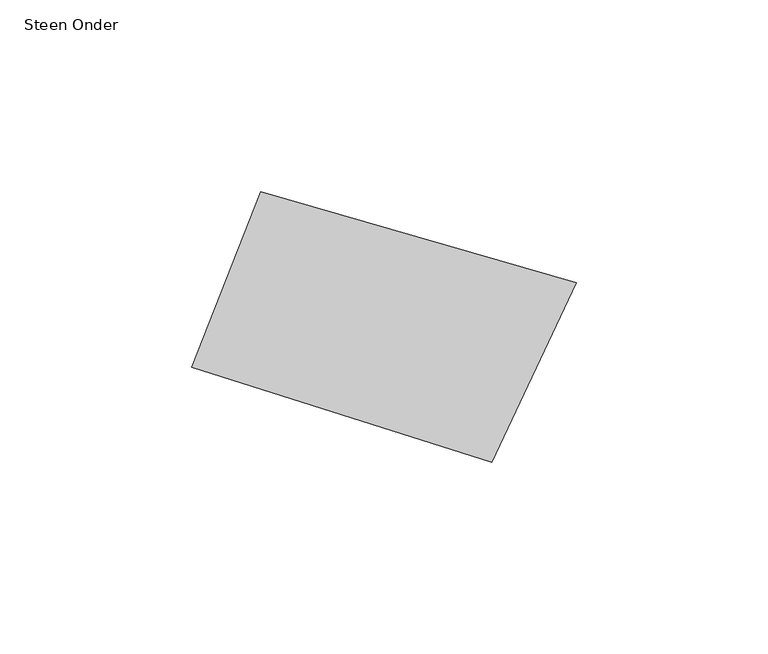
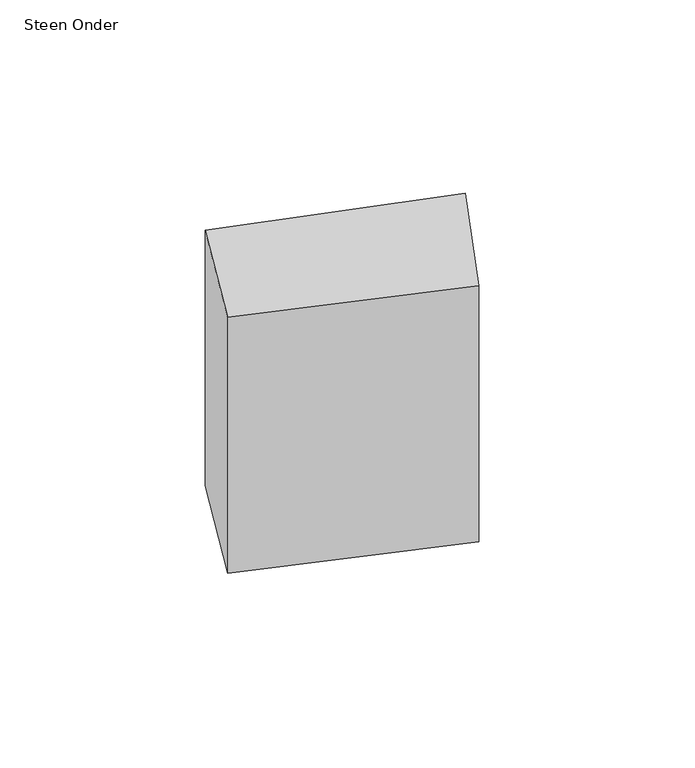
"""IFC4 building model written with IfcOpenShell, lengths in millimetres: proxy geometry, 00_GMA_steen_versie_4 : Steen Onder."""

from ifc_helpers import new_model, si_unit, frame, origin, place, context, project, spatial, polyline, outline, extrude, source, transform, mapped, element, save


def steen_onder_f78c49ac(model_context):
    return source(origin(), model_context, "Body", "SweptSolid", [
        extrude(outline(polyline([(142.4890571, 52.7339792), (120.3755051, 5.9468725), (41.9783583, 30.7378655), (60.0823517, 76.5869913), (142.4890571, 52.7339792)])), frame((0.0, 0.0, -100.0), z_axis=(0.0, 0.0, 1.0), x_axis=(1.0, 0.0, 0.0)), (0.0, 0.0, 1.0), 100.0),
    ])


if __name__ == "__main__":
    model = new_model("IFC4")
    model_context = context("Model", 3, world=origin())
    ifc_project = project(units=[si_unit("LENGTHUNIT", "METRE", prefix="MILLI")], contexts=[model_context])
    site = spatial("IfcSite", under=ifc_project)
    building = spatial("IfcBuilding", under=site)
    placement = place(None, origin())
    steen_onder_shape = steen_onder_f78c49ac(model_context)
    element("IfcBuildingElementProxy", 1, Name="00_GMA_steen_versie_4 : Steen Onder", ObjectType="00_GMA_steen_versie_4 : Steen Onder", at=placement, inside=building, context=model_context, shape_type="MappedRepresentation", body=[
        mapped(steen_onder_shape, transform((0.0, 0.0, 0.0), x_axis=(1.0, 0.0, 0.0), y_axis=(0.0, 1.0, 0.0), z_axis=(0.0, 0.0, 1.0))),
    ])
    save(model, "model.ifc")

# Revit data of these elements
# Type "00_GMA_steen_versie_4 : Steen Onder"
#   StootVoegHalfBoven [instance default] = 5 mm
#   StootVoegHalf [instance default] = 5 mm
#   StootVoegBreedteOnder = 10 mm
#   StootVoegBreedteBoven = 10 mm
#   Steendikte = 100 mm
#   LintVoegOnderHalf = 0 mm
#   LintVoegOnder = 0 mm
#   LintVoegBovenHalf = 5 mm
#   LintVoegBoven = 10 mm
#   materiaal = none
#   MateriaalVoeg = none
#   Default Elevation = 0
